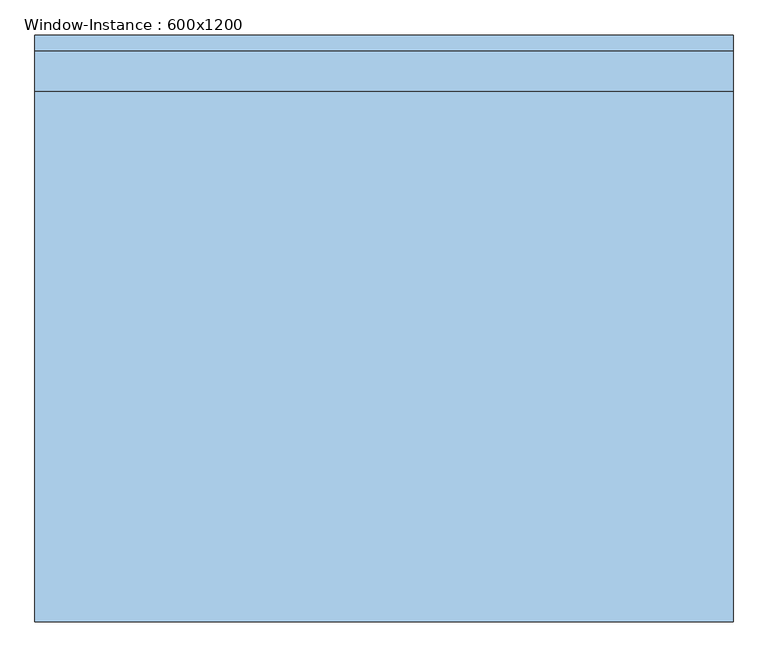
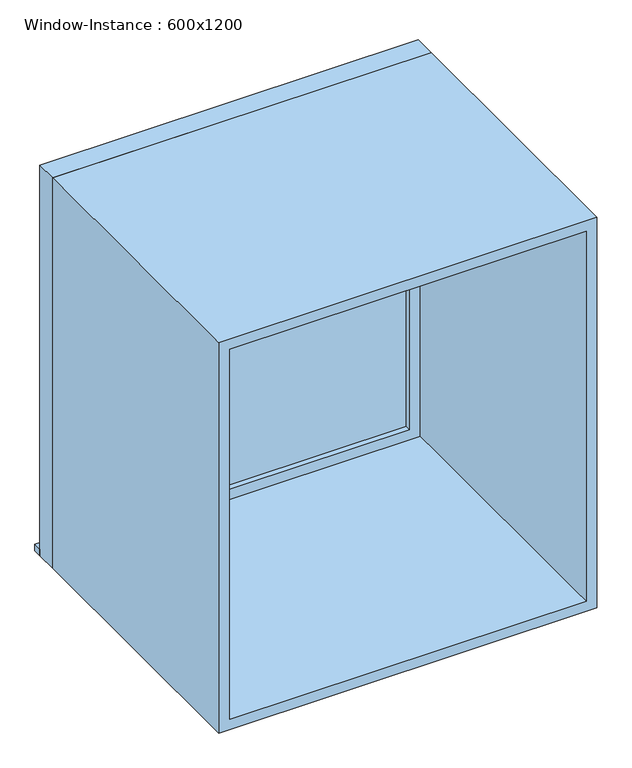
"""IFC4 building model written with IfcOpenShell, lengths in millimetres: window geometry, Window-Instance : 600x1200."""

from ifc_helpers import new_model, si_unit, frame, origin, place, context, project, spatial, polyline, outline, extrude, source, transform, mapped, element, save


def window_instance_600x1200_97efc211(model_context):
    return source(origin(), model_context, "Body", "SweptSolid", [
        extrude(outline(polyline([(-588.1, 475.4), (511.9, 475.4), (511.9, 450.0), (-588.1, 450.0), (-588.1, 475.4)])), frame((0.0, 0.0, 900.0), z_axis=(0.0, 0.0, 1.0), x_axis=(1.0, 0.0, 0.0)), (0.0, 0.0, 1.0), 19.05),
        extrude(outline(polyline([(448.4, 401.425), (-524.6, 401.425), (-524.6, 414.125), (448.4, 414.125), (448.4, 401.425)])), frame((0.0, 0.0, 963.5), z_axis=(0.0, 0.0, 1.0), x_axis=(1.0, 0.0, 0.0)), (0.0, 0.0, 1.0), 1073.0),
        extrude(outline(polyline([(2080.95, -569.05), (919.05, -569.05), (919.05, 492.85), (2080.95, 492.85), (2080.95, -569.05)]), holes=[polyline([(2036.5, -524.6), (2036.5, 448.4), (963.5, 448.4), (963.5, -524.6), (2036.5, -524.6)])]), frame((0.0, 385.55, 0.0), z_axis=(0.0, 1.0, 0.0), x_axis=(0.0, 0.0, 1.0)), (0.0, 0.0, 1.0), 44.45),
        extrude(outline(polyline([(2100.0, -588.1), (900.0, -588.1), (900.0, 511.9), (2100.0, 511.9), (2100.0, -588.1)]), holes=[polyline([(2068.25, -556.35), (2068.25, 480.15), (931.75, 480.15), (931.75, -556.35), (2068.25, -556.35)])]), frame((0.0, -450.0, 0.0), z_axis=(0.0, 1.0, 0.0), x_axis=(0.0, 0.0, 1.0)), (0.0, 0.0, 1.0), 835.55),
        extrude(outline(polyline([(2100.0, 511.9), (2100.0, -588.1), (900.0, -588.1), (900.0, 511.9), (2100.0, 511.9)]), holes=[polyline([(2080.95, 492.85), (919.05, 492.85), (919.05, -569.05), (2080.95, -569.05), (2080.95, 492.85)])]), frame((0.0, 385.55, 0.0), z_axis=(0.0, 1.0, 0.0), x_axis=(0.0, 0.0, 1.0)), (0.0, 0.0, 1.0), 64.45),
    ])


if __name__ == "__main__":
    model = new_model("IFC4")
    model_context = context("Model", 3, world=origin())
    ifc_project = project(units=[si_unit("LENGTHUNIT", "METRE", prefix="MILLI")], contexts=[model_context])
    site = spatial("IfcSite", under=ifc_project)
    building = spatial("IfcBuilding", under=site)
    placement = place(None, origin())
    window_instance_600x1200_shape = window_instance_600x1200_97efc211(model_context)
    element("IfcWindow", 1, ObjectType="Window-Instance : 600x1200", at=placement, inside=building, context=model_context, shape_type="MappedRepresentation", body=[
        mapped(window_instance_600x1200_shape, transform((0.0, 0.0, 0.0), x_axis=(1.0, 0.0, 0.0), y_axis=(0.0, 1.0, 0.0), z_axis=(0.0, 0.0, 1.0))),
    ])
    save(model, "model.ifc")

# Revit data of these elements
# Type "Window-Instance : 600x1200"
#   Type Mark = "7"
#   Construction Type Id = "GSP4R"
#   Assembly Code = "B2020100"
#   Analytic Construction = "1/8 in Pilkington single glazing"
#   Visual Light Transmittance = 0.9
#   Thermal Resistance (R) = 0.149095 (m²·K)/W
#   Solar Heat Gain Coefficient = 0.86
#   Heat Transfer Coefficient (U) = 6.70716 W/(m²·K)
#   Height [instance default] = 1200 mm
#   Default Sill Height = 900 mm
#   Width [instance default] = 600 mm
#   Window Inset = 20 mm
#   Glass Pane Material = WW-EC-GL-Storefront
#   Sash Material = WW-EC-RGB-White
#   Wall Closure = (empty or 0)
# Element 1 (IfcWindow, "Window-Instance : 600x1200")
#   Width = 1100 mm
#   Materials on its faces: "WW-EC-RGB-White", "WW-EC-GL-Storefront"
# Materials
#   "WW-EC-GL-Storefront": class "Glass", colour RGB 236 240 239, transparency 0.85, Description = "Storefront Glass", Cost = 0
#   "WW-EC-RGB-White": class "Generic", colour RGB 255 255 255, transparency 0, Comments = "If region requests off-white, swith asset color to RGB 231-228-220", Description = "Generic Color", Cost = 0
